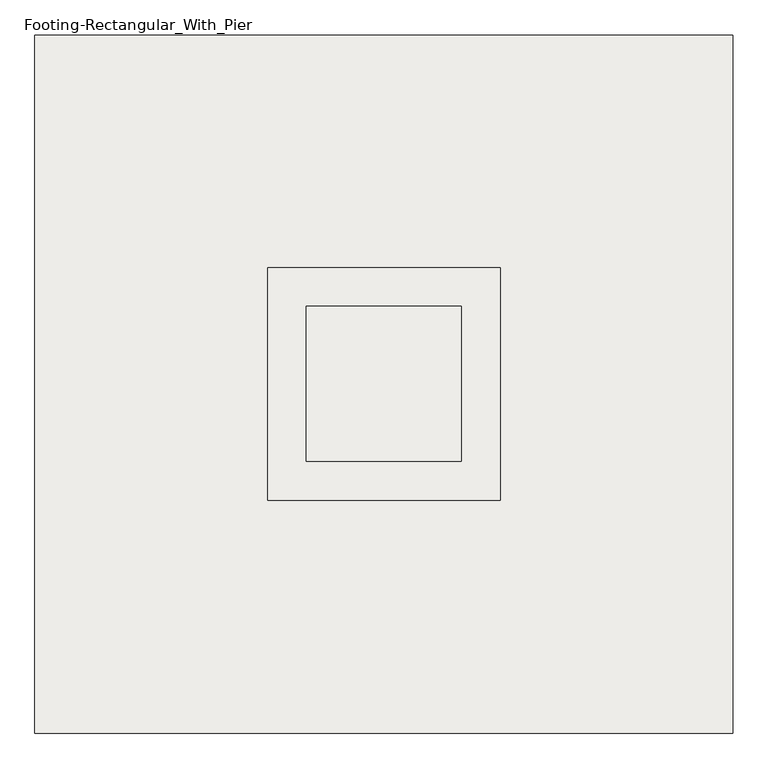
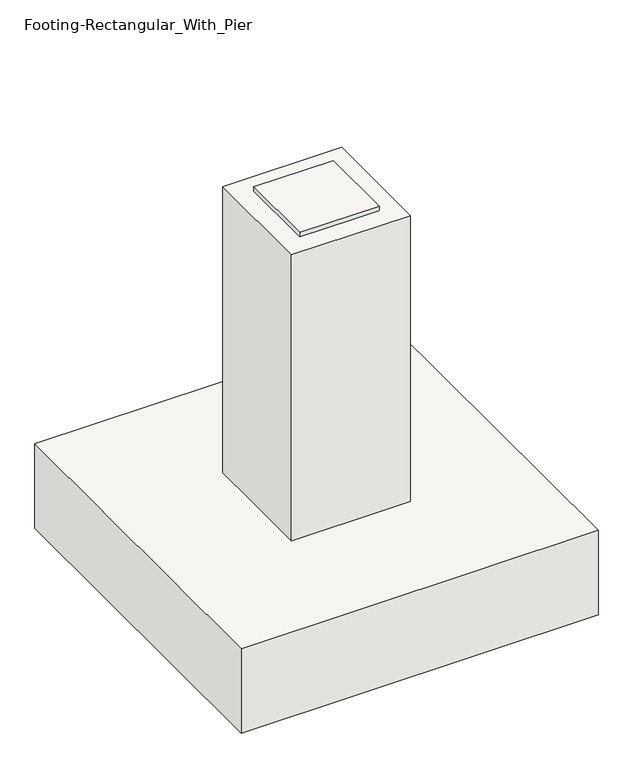
"""IFC4 building model written with IfcOpenShell, lengths in millimetres: slab geometry, Footing-Rectangular_With_Pier."""

import ifcopenshell
import ifcopenshell.guid

model = None  # the IFC model being written
_history = None  # IfcOwnerHistory: only IFC2X3 demands one
_inside = {}  # id of a spatial element -> (the spatial element, [elements in it])
_under = {}  # id of a project, library or spatial element -> (it, [spatial elements below it])
_declared = {}  # id of a project -> (the project, [libraries it declares])
_typed = {}  # id of a type object -> (the type object, [elements of that type])
_made_of = {}  # id of a material, layer set ... -> (it, [elements and type objects made of it])


def new_model(schema):
    """Start an empty IFC model of exactly this schema.

    Asked for "IFC4X3", IfcOpenShell would pick the latest addendum, in which some entities
    have other attributes; the version numbers below select the first issue.
    IFC2X3 requires an IfcOwnerHistory on every rooted entity: one is made here for all.
    """
    global model, _history
    if schema == "IFC4X3":
        model = ifcopenshell.file(schema_version=(4, 3, 0, 0))
    else:
        model = ifcopenshell.file(schema=schema)
    _inside.clear()
    _under.clear()
    _declared.clear()
    _typed.clear()
    _made_of.clear()
    _history = None
    if model.schema == "IFC2X3":
        org = make("IfcOrganization", Name="unknown")
        user = make(
            "IfcPersonAndOrganization",
            ThePerson=make("IfcPerson", FamilyName="unknown"),
            TheOrganization=org,
        )
        app = make(
            "IfcApplication",
            ApplicationDeveloper=org,
            Version="unknown",
            ApplicationFullName="unknown",
            ApplicationIdentifier="unknown",
        )
        _history = make(
            "IfcOwnerHistory",
            OwningUser=user,
            OwningApplication=app,
            ChangeAction="ADDED",
            CreationDate=0,
        )
    return model


def make(cls, **values):
    """One entity of the class cls with the attributes given. An attribute that is None is left unset."""
    return model.create_entity(
        cls, **{name: value for name, value in values.items() if value is not None}
    )


def rooted(cls, **values):
    """An entity with a GlobalId (a new one), such as an element, a storey or a relation."""
    return make(cls, GlobalId=ifcopenshell.guid.new(), OwnerHistory=_history, **values)


def si_unit(unit_type, name, prefix=None):
    """IfcSIUnit, for example si_unit("LENGTHUNIT", "METRE", prefix="MILLI")."""
    return make("IfcSIUnit", UnitType=unit_type, Prefix=prefix, Name=name)


def assignment(units):
    """IfcUnitAssignment: the units of a project."""
    return None if units is None else make("IfcUnitAssignment", Units=units)


def point(xyz):
    """IfcCartesianPoint."""
    return None if xyz is None else make("IfcCartesianPoint", Coordinates=xyz)


def direction(xyz):
    """IfcDirection."""
    return None if xyz is None else make("IfcDirection", DirectionRatios=xyz)


def frame(location, z_axis=None, x_axis=None):
    """IfcAxis2Placement3D, a coordinate frame: its origin and axes. An axis left out is left unset."""
    return make(
        "IfcAxis2Placement3D",
        Location=point(location),
        Axis=direction(z_axis),
        RefDirection=direction(x_axis),
    )


def origin():
    """The frame at (0, 0, 0) with its axes left unset."""
    return frame((0.0, 0.0, 0.0))


def origin_with_axes():
    """The frame at (0, 0, 0) with the z axis (0, 0, 1) and the x axis (1, 0, 0) written out."""
    return frame((0.0, 0.0, 0.0), z_axis=(0.0, 0.0, 1.0), x_axis=(1.0, 0.0, 0.0))


def place(relative_to, where):
    """IfcLocalPlacement: puts the frame where relative to a parent placement (None: the world)."""
    return make(
        "IfcLocalPlacement", PlacementRelTo=relative_to, RelativePlacement=where
    )


def context(
    kind, dimensions, precision=None, world=None, true_north=None, identifier=None
):
    """IfcGeometricRepresentationContext, for example the 3D "Model" context."""
    return make(
        "IfcGeometricRepresentationContext",
        ContextIdentifier=identifier,
        ContextType=kind,
        CoordinateSpaceDimension=dimensions,
        Precision=precision,
        WorldCoordinateSystem=world,
        TrueNorth=true_north,
    )


def project(units=None, contexts=None):
    """IfcProject with its units and contexts."""
    return rooted(
        "IfcProject",
        Name="project",
        RepresentationContexts=contexts,
        UnitsInContext=assignment(units),
    )


def spatial(cls, under=None, at=None, **own):
    """A site, building, storey or space (cls), placed at a placement, below another one or the project."""
    s = rooted(cls, ObjectPlacement=at, **own)
    if under is not None:
        _under.setdefault(under.id(), (under, []))[1].append(s)
    return s


def polyline(points):
    """IfcPolyline through the points."""
    return make("IfcPolyline", Points=[point(p) for p in points])


def outline(outer, holes=None, kind="AREA"):
    """IfcArbitraryClosedProfileDef: a profile drawn as a closed curve; with holes, ...WithVoids."""
    if holes is None:
        return make("IfcArbitraryClosedProfileDef", ProfileType=kind, OuterCurve=outer)
    return make(
        "IfcArbitraryProfileDefWithVoids",
        ProfileType=kind,
        OuterCurve=outer,
        InnerCurves=holes,
    )


def extrude(swept, where, along, depth):
    """IfcExtrudedAreaSolid: the profile swept, set in the frame where, extruded along a direction by depth."""
    return make(
        "IfcExtrudedAreaSolid",
        SweptArea=swept,
        Position=where,
        ExtrudedDirection=direction(along),
        Depth=depth,
    )


def shape(context_of_items, identifier, shape_type, items):
    """IfcShapeRepresentation: the items that make up one representation, for example the "Body"."""
    return make(
        "IfcShapeRepresentation",
        ContextOfItems=context_of_items,
        RepresentationIdentifier=identifier,
        RepresentationType=shape_type,
        Items=items,
    )


def source(mapping_origin, context_of_items, identifier, shape_type, items):
    """IfcRepresentationMap: a shape defined once, which mapped items show again and again."""
    return make(
        "IfcRepresentationMap",
        MappingOrigin=mapping_origin,
        MappedRepresentation=shape(context_of_items, identifier, shape_type, items),
    )


def transform(
    local_origin,
    x_axis=None,
    y_axis=None,
    z_axis=None,
    scale=None,
    scale2=None,
    scale3=None,
    uniform=True,
):
    """IfcCartesianTransformationOperator3D, or its non-uniform kind. x_axis, y_axis, z_axis: its Axis1, 2, 3."""
    if uniform:
        return make(
            "IfcCartesianTransformationOperator3D",
            Axis1=direction(x_axis),
            Axis2=direction(y_axis),
            LocalOrigin=point(local_origin),
            Scale=scale,
            Axis3=direction(z_axis),
        )
    return make(
        "IfcCartesianTransformationOperator3DnonUniform",
        Axis1=direction(x_axis),
        Axis2=direction(y_axis),
        LocalOrigin=point(local_origin),
        Scale=scale,
        Axis3=direction(z_axis),
        Scale2=scale2,
        Scale3=scale3,
    )


def mapped(mapping_source, mapping_target):
    """IfcMappedItem: shows the shape of a source again, moved by a transform."""
    return make(
        "IfcMappedItem", MappingSource=mapping_source, MappingTarget=mapping_target
    )


def made_of(thing, what):
    """Note that an element or type object is made of a material, layer set ...; save() writes the relation."""
    if what is not None:
        _made_of.setdefault(what.id(), (what, []))[1].append(thing)
    return thing


def element(
    cls,
    number,
    at=None,
    inside=None,
    cuts=None,
    type_object=None,
    material=None,
    context=None,
    identifier="Body",
    shape_type=None,
    held_by="IfcProductDefinitionShape",
    body=None,
    shapes=None,
    **own,
):
    """One element of the class cls, such as IfcWall. Its Tag is "e" and its number.

    at: its placement. inside: the storey or other place that contains it. cuts: it is an
    opening in that element (IfcRelVoidsElement). A single representation is given by context,
    identifier, shape_type and body (its items); several are given by shapes. held_by: the class
    of the entity that holds the representations. save() writes the other relations.
    """
    e = rooted(cls, Tag="e%d" % number, ObjectPlacement=at, **own)
    if body is not None:
        shapes = [shape(context, identifier, shape_type, body)]
    if shapes is not None:
        e.Representation = make(held_by, Representations=shapes)
    if inside is not None:
        _inside.setdefault(inside.id(), (inside, []))[1].append(e)
    if cuts is not None:
        rooted(
            "IfcRelVoidsElement", RelatingBuildingElement=cuts, RelatedOpeningElement=e
        )
    if type_object is not None:
        _typed.setdefault(type_object.id(), (type_object, []))[1].append(e)
    return made_of(e, material)


def aggregate(whole, parts):
    """IfcRelAggregates: a whole, such as a stair, and the parts it consists of."""
    return rooted("IfcRelAggregates", RelatingObject=whole, RelatedObjects=parts)


def save(model, path):
    """Write the relations noted so far, then the file.

    IfcRelAggregates (storeys below a building ...), IfcRelContainedInSpatialStructure (elements
    in a storey), IfcRelDefinesByType, IfcRelAssociatesMaterial and IfcRelDeclares: one each for
    every whole, place, type object, material and project.
    """
    for whole, parts in _under.values():
        aggregate(whole, parts)
    for where, things in _inside.values():
        rooted(
            "IfcRelContainedInSpatialStructure",
            RelatedElements=things,
            RelatingStructure=where,
        )
    for kind, things in _typed.values():
        rooted("IfcRelDefinesByType", RelatedObjects=things, RelatingType=kind)
    for what, things in _made_of.values():
        rooted("IfcRelAssociatesMaterial", RelatedObjects=things, RelatingMaterial=what)
    for by, libraries in _declared.values():
        rooted("IfcRelDeclares", RelatingContext=by, RelatedDefinitions=libraries)
    model.write(path)


def footing_rectangular_with_pier_e052c68f(model_context):
    return source(origin(), model_context, "Body", "SweptSolid", [
        extrude(outline(polyline([(203.2, 203.2), (203.2, -203.2), (-203.2, -203.2), (-203.2, 203.2), (203.2, 203.2)])), frame((0.0, 0.0, 1549.4), z_axis=(0.0, 0.0, 1.0), x_axis=(1.0, 0.0, 0.0)), (0.0, 0.0, 1.0), 25.4),
        extrude(outline(polyline([(914.4, 914.4), (914.4, -914.4), (-914.4, -914.4), (-914.4, 914.4), (914.4, 914.4)])), frame((0.0, 0.0, -457.2), z_axis=(0.0, 0.0, 1.0), x_axis=(1.0, 0.0, 0.0)), (0.0, 0.0, 1.0), 457.2),
        extrude(outline(polyline([(304.8, 304.8), (304.8, -304.8), (-304.8, -304.8), (-304.8, 304.8), (304.8, 304.8)])), origin_with_axes(), (0.0, 0.0, 1.0), 1549.4),
    ])


if __name__ == "__main__":
    model = new_model("IFC4")
    model_context = context("Model", 3, world=origin())
    ifc_project = project(units=[si_unit("LENGTHUNIT", "METRE", prefix="MILLI")], contexts=[model_context])
    site = spatial("IfcSite", under=ifc_project)
    building = spatial("IfcBuilding", under=site)
    placement = place(None, origin())
    footing_rectangular_with_pier_shape = footing_rectangular_with_pier_e052c68f(model_context)
    element("IfcSlab", 1, ObjectType="Footing-Rectangular_With_Pier : F3 - 6'-0\" x 6'-0\" x 1'-6\"", at=placement, inside=building, context=model_context, shape_type="MappedRepresentation", body=[
        mapped(footing_rectangular_with_pier_shape, transform((0.0, 0.0, 0.0), x_axis=(1.0, 0.0, 0.0), y_axis=(0.0, 1.0, 0.0), z_axis=(0.0, 0.0, 1.0))),
    ])
    save(model, "model.ifc")

# Revit data of these elements
# Type "Footing-Rectangular_With_Pier : F3 - 6'-0\" x 6'-0\" x 1'-6\""
#   Type Mark = "F3"
#   Assembly Code = "A1010100"
#   Width = 1828.8 mm
#   SteelPlateWidth [instance default] = 406.4 mm
#   SteelPlateThickness [instance default] = 25.4 mm
#   SteelPlateDepth [instance default] = 406.4 mm
#   PierWidth [instance default] = 609.6 mm
#   PierLength [instance default] = 609.6 mm
#   PierDepth [instance default] = 1371.6 mm
#   Length = 1828.8 mm
#   FootingThickness = 457.2 mm
#   Steel Plate = yes
#   Structural Material [instance default] = Concrete - Cast-in-Place Concrete
# Element 1 (IfcSlab, "Footing-Rectangular_With_Pier : F3 - 6'-0\" x 6'-0\" x 1'-6\"")
#   PierDepth = 1549.4 mm
#   Materials on its faces: "Concrete - Cast-in-Place Concrete", "Steel"
# Materials
#   "Concrete - Cast-in-Place Concrete": class "Concrete", colour RGB 192 192 192, transparency 0
#   "Steel": class "Metal", colour RGB 247 247 247, transparency 0, Description = "Steel, mill finish", Cost = 0
